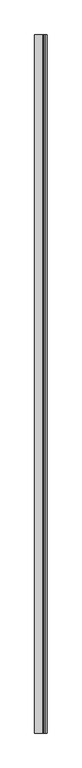
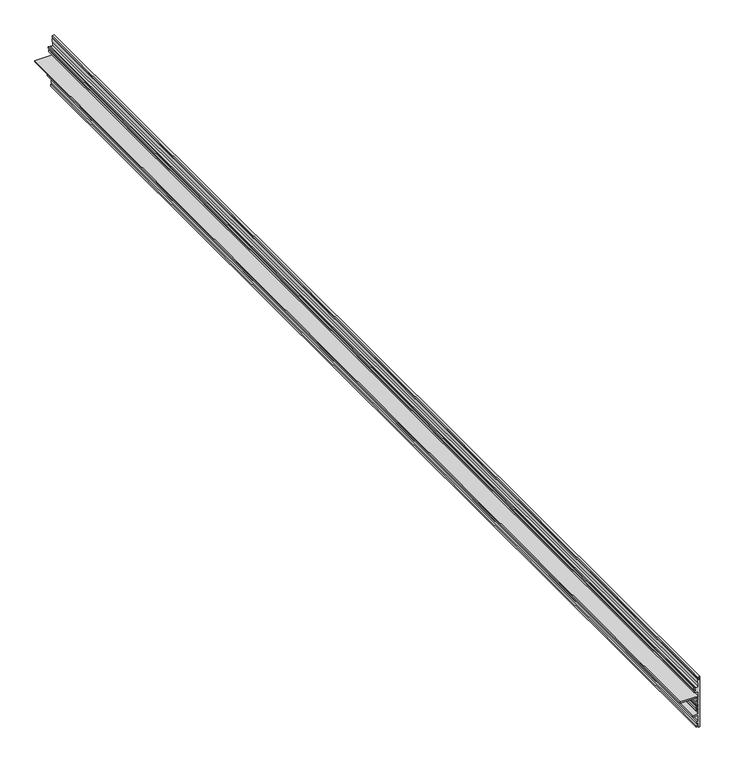
"""IFC4 building model written with IfcOpenShell, lengths in millimetres: proxy geometry, Door frame12:Door frame003:296356 : Door frame12:Door frame003:296356."""

from ifc_helpers import new_model, si_unit, frame, origin, place, context, project, spatial, polyline, outline, extrude, source, transform, mapped, element, save


def generic_models_fc56faae(model_context):
    return source(origin(), model_context, "Body", "SweptSolid", [
        extrude(outline(polyline([(36640.7292623, 20333.6451942), (36640.7292623, 20335.8033351), (36638.6348329, 20335.8033351), (36638.6348329, 20332.2468048), (36635.0786991, 20332.2468048), (36635.0786991, 20333.6440533), (36637.237374, 20333.6440533), (36637.237374, 20335.8024221), (36629.3636227, 20335.8024221), (36629.3636227, 20333.643193), (36631.522833, 20333.643193), (36631.522833, 20332.2457341), (36627.9663742, 20332.2457341), (36627.9663742, 20335.8016404), (36625.8711226, 20335.8016404), (36625.8711226, 20333.6451942), (36624.9183358, 20331.7403376), (36623.9664094, 20333.645481), (36623.9664094, 20335.8016239), (36617.0240434, 20335.8016239), (36617.0240434, 20326.0194939), (36613.8490434, 20326.0194939), (36613.8490434, 20335.7984939), (36602.905231, 20335.7984939), (36602.905231, 20333.3106739), (36598.5961003, 20333.3106739), (36600.1211436, 20335.8099419), (36594.775583, 20335.8099419), (36595.6482078, 20332.5532616), (36592.4137824, 20332.2698838), (36593.5561506, 20334.6097431), (36593.5561506, 20335.9679638), (36591.6240434, 20335.9679638), (36591.6240434, 20338.9855213), (36686.8713846, 20338.9855213), (36686.8713846, 20334.8605056), (36684.2230088, 20334.8605056), (36684.2230088, 20336.1151812), (36685.5545864, 20336.1151812), (36685.5545864, 20337.600201), (36680.6298938, 20337.600201), (36680.6298938, 20336.1151812), (36681.9249044, 20336.1151812), (36681.9249044, 20334.8605056), (36675.7714394, 20334.8605056), (36675.7714394, 20336.0617223), (36667.7720071, 20336.0617223), (36667.7720071, 20331.3652798), (36667.5392258, 20330.1662269), (36668.6824408, 20327.8267117), (36665.4469498, 20328.1093782), (36666.3193526, 20331.3652299), (36660.9960694, 20331.3652299), (36662.4395074, 20328.865122), (36658.8017047, 20328.865122), (36658.8017047, 20335.8052001), (36650.6101085, 20335.8052001), (36650.6101085, 20304.0605156), (36648.0323358, 20304.0605156), (36648.0323358, 20335.804496), (36642.634549, 20335.804496), (36642.634549, 20333.645481), (36641.6823358, 20331.7403376), (36640.7292623, 20333.6451942)])), frame((0.0, -774.5581156, 0.0), z_axis=(0.0, 1.0, 0.0), x_axis=(0.0, 0.0, 1.0)), (0.0, 0.0, 1.0), 1999.85),
    ])


if __name__ == "__main__":
    model = new_model("IFC4")
    model_context = context("Model", 3, world=origin())
    ifc_project = project(units=[si_unit("LENGTHUNIT", "METRE", prefix="MILLI")], contexts=[model_context])
    site = spatial("IfcSite", under=ifc_project)
    building = spatial("IfcBuilding", under=site)
    placement = place(None, origin())
    generic_models_shape = generic_models_fc56faae(model_context)
    element("IfcBuildingElementProxy", 1, Name="Door frame12:Door frame003:296356 : Door frame12:Door frame003:296356", ObjectType="Door frame12:Door frame003:296356 : Door frame12:Door frame003:296356", at=placement, inside=building, context=model_context, shape_type="MappedRepresentation", body=[
        mapped(generic_models_shape, transform((0.0, 0.0, 0.0), x_axis=(1.0, 0.0, 0.0), y_axis=(0.0, 1.0, 0.0), z_axis=(0.0, 0.0, 1.0))),
    ])
    save(model, "model.ifc")

# Revit data of these elements
# Type "Door frame12:Door frame003:296356 : Door frame12:Door frame003:296356"
#   NameOverride = "Door frame12:Door frame003:296356"
#   ObjectTypeOverride = "Door frame12:Door frame003"
#   Reference = "Door frame003"
#   Category = "Generic Models"
#   Tag = "296356"
# Element 1 (IfcBuildingElementProxy, "Door frame12:Door frame003:296356 : Door frame12:Door frame003:296356")
#   Materials on its faces: "FLEETWOOD SERIES T-3200 SINGLE SWING DOOR FRAME"
# Materials
#   "FLEETWOOD SERIES T-3200 SINGLE SWING DOOR FRAME": class "Unassigned", colour RGB 128 128 128, transparency 0, Cost = 0
